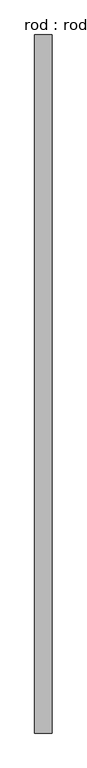
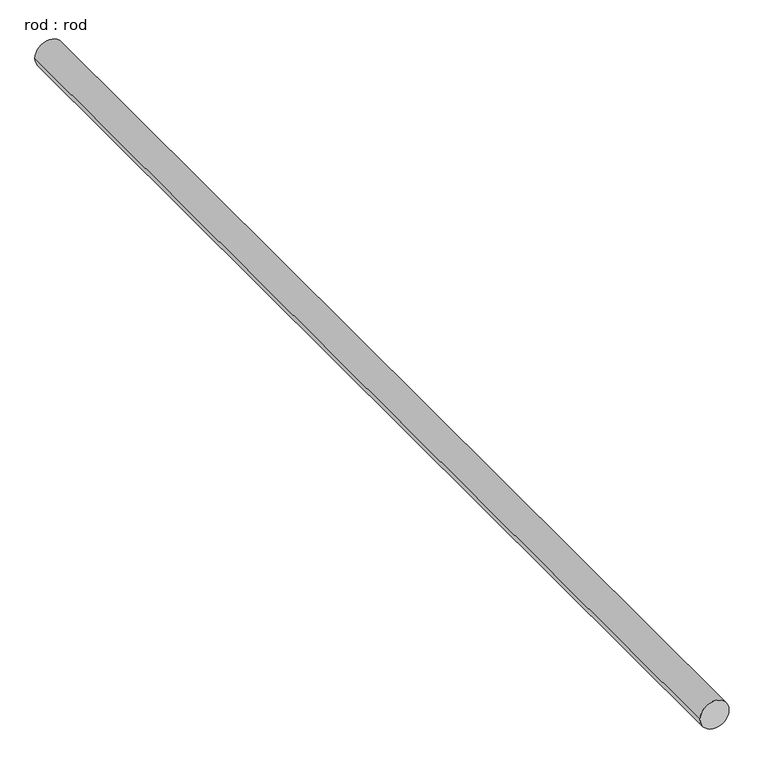
"""IFC4 building model written with IfcOpenShell, lengths in millimetres: proxy geometry, rod : rod."""

from ifc_helpers import new_model, si_unit, point, frame, frame_2d, origin, place, context, project, spatial, circle_curve, trimmed, segment, composite_curve, outline, extrude, source, transform, mapped, element, save


def rod_rod_4c3c0aff(model_context):
    return source(origin(), model_context, "Body", "SweptSolid", [
        extrude(outline(composite_curve([segment(trimmed(circle_curve(frame_2d((0.0108462, 0.0)), 200.0), [point((0.0108462, 200.0))], [point((0.0108462, -200.0))], False, "CARTESIAN"), True, "CONTINUOUS"), segment(trimmed(circle_curve(frame_2d((0.0108462, 0.0)), 200.0), [point((0.0108462, -200.0))], [point((0.0108462, 200.0))], False, "CARTESIAN"), True, "CONTINUOUS")], self_intersect=False)), frame((0.0, -3854.9093248, 0.0), z_axis=(0.0, 1.0, 0.0), x_axis=(0.0, 0.0, 1.0)), (0.0, 0.0, 1.0), 15895.2758804),
    ])


if __name__ == "__main__":
    model = new_model("IFC4")
    model_context = context("Model", 3, world=origin())
    ifc_project = project(units=[si_unit("LENGTHUNIT", "METRE", prefix="MILLI")], contexts=[model_context])
    site = spatial("IfcSite", under=ifc_project)
    building = spatial("IfcBuilding", under=site)
    placement = place(None, origin())
    rod_rod_shape = rod_rod_4c3c0aff(model_context)
    element("IfcBuildingElementProxy", 1, Name="rod : rod", ObjectType="rod : rod", at=placement, inside=building, context=model_context, shape_type="MappedRepresentation", body=[
        mapped(rod_rod_shape, transform((0.0, 0.0, 0.0), x_axis=(1.0, 0.0, 0.0), y_axis=(0.0, 1.0, 0.0), z_axis=(0.0, 0.0, 1.0))),
    ])
    save(model, "model.ifc")

# Revit data of these elements
# Type "rod : rod"
#   Default Elevation = 0
